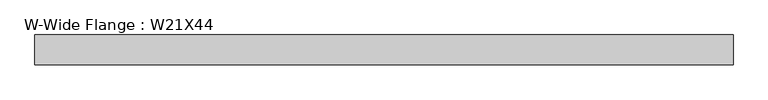
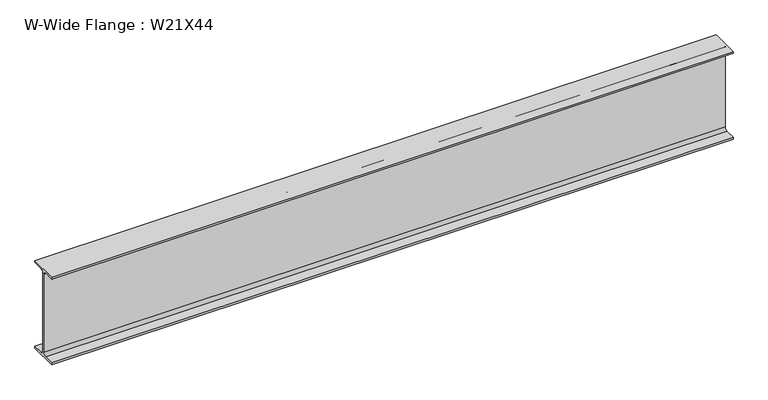
"""IFC4 building model written with IfcOpenShell, lengths in millimetres: beam geometry, W-Wide Flange : W21X44."""

from ifc_helpers import new_model, si_unit, point, frame, frame_2d, origin, place, context, project, spatial, polyline, circle_curve, trimmed, segment, composite_curve, outline, extrude, source, transform, mapped, element, save


def w_wide_flange_w21x44_b9bda158(model_context):
    return source(origin(), model_context, "Body", "SweptSolid", [
        extrude(outline(composite_curve([segment(polyline([(82.55, -251.46), (82.55, -262.89), (-82.55, -262.89), (-82.55, -251.46), (-21.59, -251.46)]), True, "CONTINUOUS"), segment(trimmed(circle_curve(frame_2d((-21.59, -234.315)), 17.145), [point((-21.59, -251.46))], [point((-4.445, -234.315))], True, "CARTESIAN"), True, "CONTINUOUS"), segment(polyline([(-4.445, -234.315), (-4.445, 234.315)]), True, "CONTINUOUS"), segment(trimmed(circle_curve(frame_2d((-21.59, 234.315)), 17.145), [point((-4.445, 234.315))], [point((-21.59, 251.46))], True, "CARTESIAN"), True, "CONTINUOUS"), segment(polyline([(-21.59, 251.46), (-82.55, 251.46), (-82.55, 262.89), (82.55, 262.89), (82.55, 251.46), (21.59, 251.46)]), True, "CONTINUOUS"), segment(trimmed(circle_curve(frame_2d((21.59, 234.315)), 17.145), [point((21.59, 251.46))], [point((4.445, 234.315))], True, "CARTESIAN"), True, "CONTINUOUS"), segment(polyline([(4.445, 234.315), (4.445, -234.315)]), True, "CONTINUOUS"), segment(trimmed(circle_curve(frame_2d((21.59, -234.315)), 17.145), [point((4.445, -234.315))], [point((21.59, -251.46))], True, "CARTESIAN"), True, "CONTINUOUS"), segment(polyline([(21.59, -251.46), (82.55, -251.46)]), True, "CONTINUOUS")], self_intersect=False)), frame((-1935.665346, 0.0, 0.0), z_axis=(1.0, 0.0, 0.0), x_axis=(0.0, 1.0, 0.0)), (0.0, 0.0, 1.0), 3868.155692),
    ])


if __name__ == "__main__":
    model = new_model("IFC4")
    model_context = context("Model", 3, world=origin())
    ifc_project = project(units=[si_unit("LENGTHUNIT", "METRE", prefix="MILLI")], contexts=[model_context])
    site = spatial("IfcSite", under=ifc_project)
    building = spatial("IfcBuilding", under=site)
    placement = place(None, origin())
    w_wide_flange_w21x44_shape = w_wide_flange_w21x44_b9bda158(model_context)
    element("IfcBeam", 1, ObjectType="W-Wide Flange : W21X44", at=placement, inside=building, context=model_context, shape_type="MappedRepresentation", body=[
        mapped(w_wide_flange_w21x44_shape, transform((0.0, 0.0, 0.0), x_axis=(1.0, 0.0, 0.0), y_axis=(0.0, 1.0, 0.0), z_axis=(0.0, 0.0, 1.0))),
    ])
    save(model, "model.ifc")

# Revit data of these elements
# Type "W-Wide Flange : W21X44"
#   Assembly Code = "B10"
#   W = 44
#   Start Extension Calculation [instance default] = 10' - 0"
#   Start Extension [instance default] = -0' - 0 1/2"
#   End Extension Calculation [instance default] = 10' - 0"
#   End Extension [instance default] = -0' - 0 1/2"
#   Length [instance default] = 5' - 0"
#   bf = 0' - 6 1/2"
#   d = 1' - 8.7"
#   k = 0' - 1 1/8"
#   k2 = 0' - 0.675"
#   tf = 0' - 0.45"
#   tw = 0' - 0.35"
#   A = 0.0902778 SF
#   Beam Material [instance default] = Metal - Steel - ASTM A992
# Element 1 (IfcBeam, "W-Wide Flange : W21X44")
#   Materials on its faces: "Metal - Steel - ASTM A992"
# Materials
#   "Metal - Steel - ASTM A992": class "Metal", colour RGB 128 0 0, transparency 0
